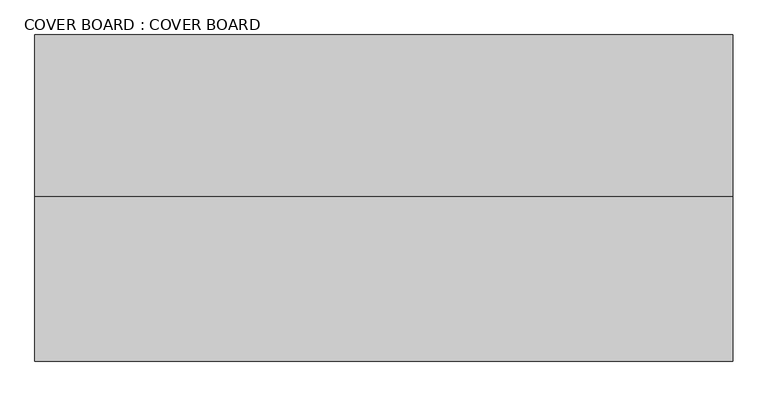
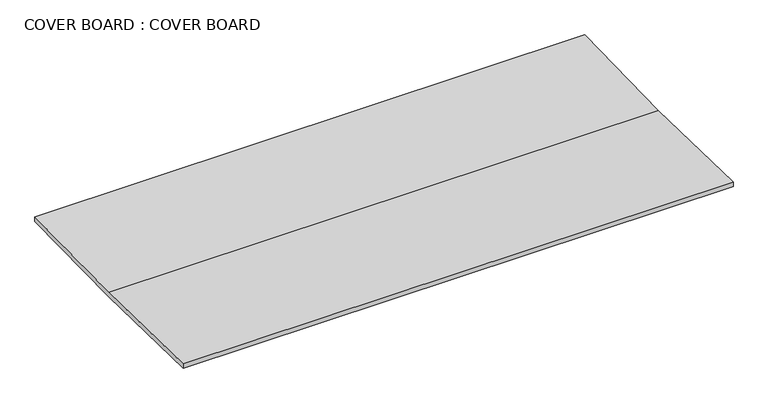
"""IFC4 building model written with IfcOpenShell, lengths in millimetres: proxy geometry, COVER BOARD : COVER BOARD."""

from ifc_helpers import new_model, si_unit, frame, origin, place, context, project, spatial, polyline, outline, extrude, source, transform, mapped, element, save


def cover_board_cover_board_90439fdb(model_context):
    return source(origin(), model_context, "Body", "SweptSolid", [
        extrude(outline(polyline([(-4872.9612169, 40211.218553), (-4408.9401513, 40221.0164062), (-4408.9401513, 40203.6846871), (-4872.9612169, 40193.8868338), (-5343.2581759, 40203.6846871), (-5343.2581759, 40221.0164063), (-4872.9612169, 40211.218553)])), frame((12382.7678845, 0.0, 0.0), z_axis=(1.0, 0.0, 0.0), x_axis=(0.0, 1.0, 0.0)), (0.0, 0.0, 1.0), 2000.0),
    ])


if __name__ == "__main__":
    model = new_model("IFC4")
    model_context = context("Model", 3, world=origin())
    ifc_project = project(units=[si_unit("LENGTHUNIT", "METRE", prefix="MILLI")], contexts=[model_context])
    site = spatial("IfcSite", under=ifc_project)
    building = spatial("IfcBuilding", under=site)
    placement = place(None, origin())
    cover_board_cover_board_shape = cover_board_cover_board_90439fdb(model_context)
    element("IfcBuildingElementProxy", 1, Name="COVER BOARD : COVER BOARD", ObjectType="COVER BOARD : COVER BOARD", at=placement, inside=building, context=model_context, shape_type="MappedRepresentation", body=[
        mapped(cover_board_cover_board_shape, transform((0.0, 0.0, 0.0), x_axis=(1.0, 0.0, 0.0), y_axis=(0.0, 1.0, 0.0), z_axis=(0.0, 0.0, 1.0))),
    ])
    save(model, "model.ifc")

# Revit data of these elements
# Type "COVER BOARD : COVER BOARD"
#   NameOverride = "COVER BOARD"
# Element 1 (IfcBuildingElementProxy, "COVER BOARD : COVER BOARD")
#   Materials on its faces: "CDX PLYWOOD - SEE STRUCTURAL DWGS"
# Materials
#   "CDX PLYWOOD - SEE STRUCTURAL DWGS": class "Unassigned", colour RGB 177 130 114, transparency 0, Cost = 0
